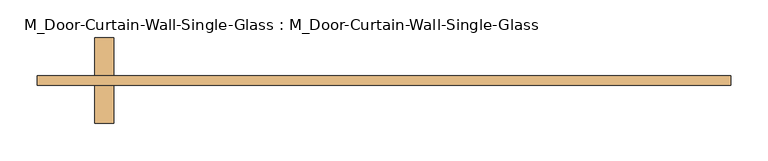
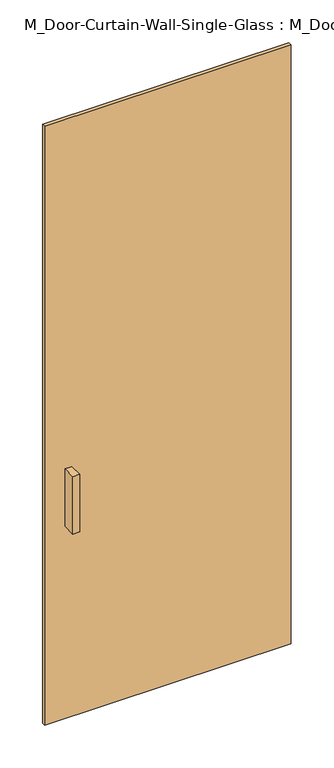
"""IFC4 building model written with IfcOpenShell, lengths in millimetres: door geometry, M_Door-Curtain-Wall-Single-Glass : M_Door-Curtain-Wall-Single-Glass."""

from ifc_helpers import new_model, si_unit, frame, origin, origin_with_axes, place, context, project, spatial, polyline, outline, extrude, source, transform, mapped, element, save


def m_door_curtain_wall_single_glass_m_door_curtain_wall_single_4acd2d97(model_context):
    return source(origin(), model_context, "Body", "SweptSolid", [
        extrude(outline(polyline([(462.5, -50.8), (-462.5, -50.8), (-462.5, -38.1), (462.5, -38.1), (462.5, -50.8)])), origin_with_axes(), (0.0, 0.0, 1.0), 2375.0),
        extrude(outline(polyline([(-360.9, 12.7), (-360.9, -38.1), (-386.3, -38.1), (-386.3, 12.7), (-360.9, 12.7)])), frame((0.0, 0.0, 762.0), z_axis=(0.0, 0.0, 1.0), x_axis=(1.0, 0.0, 0.0)), (0.0, 0.0, 1.0), 228.6),
        extrude(outline(polyline([(-386.3, -101.6), (-386.3, -50.8), (-360.9, -50.8), (-360.9, -101.6), (-386.3, -101.6)])), frame((0.0, 0.0, 762.0), z_axis=(0.0, 0.0, 1.0), x_axis=(1.0, 0.0, 0.0)), (0.0, 0.0, 1.0), 228.6),
    ])


if __name__ == "__main__":
    model = new_model("IFC4")
    model_context = context("Model", 3, world=origin())
    ifc_project = project(units=[si_unit("LENGTHUNIT", "METRE", prefix="MILLI")], contexts=[model_context])
    site = spatial("IfcSite", under=ifc_project)
    building = spatial("IfcBuilding", under=site)
    placement = place(None, origin())
    m_door_curtain_wall_single_glass_m_door_curtain_wall_single_shape = m_door_curtain_wall_single_glass_m_door_curtain_wall_single_4acd2d97(model_context)
    element("IfcDoor", 1, ObjectType="M_Door-Curtain-Wall-Single-Glass : M_Door-Curtain-Wall-Single-Glass", at=placement, inside=building, context=model_context, shape_type="MappedRepresentation", body=[
        mapped(m_door_curtain_wall_single_glass_m_door_curtain_wall_single_shape, transform((0.0, 0.0, 0.0), x_axis=(1.0, 0.0, 0.0), y_axis=(0.0, 1.0, 0.0), z_axis=(0.0, 0.0, 1.0))),
    ])
    save(model, "model.ifc")

# Revit data of these elements
# Type "M_Door-Curtain-Wall-Single-Glass : M_Door-Curtain-Wall-Single-Glass"
#   Type Mark = "50"
#   Assembly Code = "B2030100"
#   Analytic Construction = "<None>"
#   Width [instance default] = 900 mm
#   Thermal Resistance (R) = 1.7611 (m²·K)/W
#   Swing Angle [instance default] = 90.00°
#   Heat Transfer Coefficient (U) = 0.567826 W/(m²·K)
#   Offset = 50.8 mm
#   Define Thermal Properties by = 1
#   Function = 1
#   Door Handle Material = Aluminum
#   Glazing = Glass
#   Visual Light Transmittance = 0
#   Solar Heat Gain Coefficient = 0
#   Construction Type Id = ""
# Element 1 (IfcDoor, "M_Door-Curtain-Wall-Single-Glass : M_Door-Curtain-Wall-Single-Glass")
#   Width = 925 mm
#   Materials on its faces: "Aluminum", "Glass"
# Materials
#   "Aluminum": class "Metal", colour RGB 247 247 247, transparency 0, Description = "Aluminum 6061", Cost = 0
#   "Glass": class "Glass", colour RGB 0 128 192, transparency 0.9, Description = "Soda Lime Glass", Cost = 0
